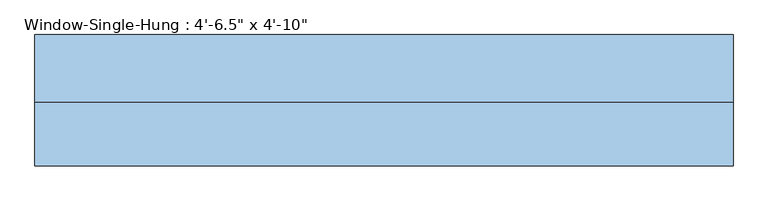
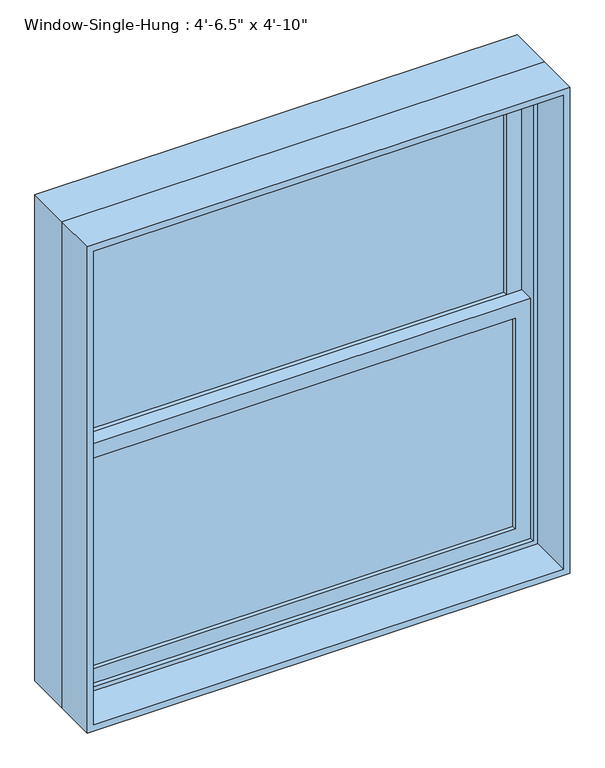
"""IFC4 building model written with IfcOpenShell, lengths in millimetres: window geometry."""

import ifcopenshell
import ifcopenshell.guid

model = None  # the IFC model being written
_history = None  # IfcOwnerHistory: only IFC2X3 demands one
_inside = {}  # id of a spatial element -> (the spatial element, [elements in it])
_under = {}  # id of a project, library or spatial element -> (it, [spatial elements below it])
_declared = {}  # id of a project -> (the project, [libraries it declares])
_typed = {}  # id of a type object -> (the type object, [elements of that type])
_made_of = {}  # id of a material, layer set ... -> (it, [elements and type objects made of it])


def new_model(schema):
    """Start an empty IFC model of exactly this schema.

    Asked for "IFC4X3", IfcOpenShell would pick the latest addendum, in which some entities
    have other attributes; the version numbers below select the first issue.
    IFC2X3 requires an IfcOwnerHistory on every rooted entity: one is made here for all.
    """
    global model, _history
    if schema == "IFC4X3":
        model = ifcopenshell.file(schema_version=(4, 3, 0, 0))
    else:
        model = ifcopenshell.file(schema=schema)
    _inside.clear()
    _under.clear()
    _declared.clear()
    _typed.clear()
    _made_of.clear()
    _history = None
    if model.schema == "IFC2X3":
        org = make("IfcOrganization", Name="unknown")
        user = make(
            "IfcPersonAndOrganization",
            ThePerson=make("IfcPerson", FamilyName="unknown"),
            TheOrganization=org,
        )
        app = make(
            "IfcApplication",
            ApplicationDeveloper=org,
            Version="unknown",
            ApplicationFullName="unknown",
            ApplicationIdentifier="unknown",
        )
        _history = make(
            "IfcOwnerHistory",
            OwningUser=user,
            OwningApplication=app,
            ChangeAction="ADDED",
            CreationDate=0,
        )
    return model


def make(cls, **values):
    """One entity of the class cls with the attributes given. An attribute that is None is left unset."""
    return model.create_entity(
        cls, **{name: value for name, value in values.items() if value is not None}
    )


def rooted(cls, **values):
    """An entity with a GlobalId (a new one), such as an element, a storey or a relation."""
    return make(cls, GlobalId=ifcopenshell.guid.new(), OwnerHistory=_history, **values)


def si_unit(unit_type, name, prefix=None):
    """IfcSIUnit, for example si_unit("LENGTHUNIT", "METRE", prefix="MILLI")."""
    return make("IfcSIUnit", UnitType=unit_type, Prefix=prefix, Name=name)


def assignment(units):
    """IfcUnitAssignment: the units of a project."""
    return None if units is None else make("IfcUnitAssignment", Units=units)


def point(xyz):
    """IfcCartesianPoint."""
    return None if xyz is None else make("IfcCartesianPoint", Coordinates=xyz)


def direction(xyz):
    """IfcDirection."""
    return None if xyz is None else make("IfcDirection", DirectionRatios=xyz)


def frame(location, z_axis=None, x_axis=None):
    """IfcAxis2Placement3D, a coordinate frame: its origin and axes. An axis left out is left unset."""
    return make(
        "IfcAxis2Placement3D",
        Location=point(location),
        Axis=direction(z_axis),
        RefDirection=direction(x_axis),
    )


def origin():
    """The frame at (0, 0, 0) with its axes left unset."""
    return frame((0.0, 0.0, 0.0))


def place(relative_to, where):
    """IfcLocalPlacement: puts the frame where relative to a parent placement (None: the world)."""
    return make(
        "IfcLocalPlacement", PlacementRelTo=relative_to, RelativePlacement=where
    )


def context(
    kind, dimensions, precision=None, world=None, true_north=None, identifier=None
):
    """IfcGeometricRepresentationContext, for example the 3D "Model" context."""
    return make(
        "IfcGeometricRepresentationContext",
        ContextIdentifier=identifier,
        ContextType=kind,
        CoordinateSpaceDimension=dimensions,
        Precision=precision,
        WorldCoordinateSystem=world,
        TrueNorth=true_north,
    )


def project(units=None, contexts=None):
    """IfcProject with its units and contexts."""
    return rooted(
        "IfcProject",
        Name="project",
        RepresentationContexts=contexts,
        UnitsInContext=assignment(units),
    )


def spatial(cls, under=None, at=None, **own):
    """A site, building, storey or space (cls), placed at a placement, below another one or the project."""
    s = rooted(cls, ObjectPlacement=at, **own)
    if under is not None:
        _under.setdefault(under.id(), (under, []))[1].append(s)
    return s


def polyline(points):
    """IfcPolyline through the points."""
    return make("IfcPolyline", Points=[point(p) for p in points])


def outline(outer, holes=None, kind="AREA"):
    """IfcArbitraryClosedProfileDef: a profile drawn as a closed curve; with holes, ...WithVoids."""
    if holes is None:
        return make("IfcArbitraryClosedProfileDef", ProfileType=kind, OuterCurve=outer)
    return make(
        "IfcArbitraryProfileDefWithVoids",
        ProfileType=kind,
        OuterCurve=outer,
        InnerCurves=holes,
    )


def extrude(swept, where, along, depth):
    """IfcExtrudedAreaSolid: the profile swept, set in the frame where, extruded along a direction by depth."""
    return make(
        "IfcExtrudedAreaSolid",
        SweptArea=swept,
        Position=where,
        ExtrudedDirection=direction(along),
        Depth=depth,
    )


def shape(context_of_items, identifier, shape_type, items):
    """IfcShapeRepresentation: the items that make up one representation, for example the "Body"."""
    return make(
        "IfcShapeRepresentation",
        ContextOfItems=context_of_items,
        RepresentationIdentifier=identifier,
        RepresentationType=shape_type,
        Items=items,
    )


def source(mapping_origin, context_of_items, identifier, shape_type, items):
    """IfcRepresentationMap: a shape defined once, which mapped items show again and again."""
    return make(
        "IfcRepresentationMap",
        MappingOrigin=mapping_origin,
        MappedRepresentation=shape(context_of_items, identifier, shape_type, items),
    )


def transform(
    local_origin,
    x_axis=None,
    y_axis=None,
    z_axis=None,
    scale=None,
    scale2=None,
    scale3=None,
    uniform=True,
):
    """IfcCartesianTransformationOperator3D, or its non-uniform kind. x_axis, y_axis, z_axis: its Axis1, 2, 3."""
    if uniform:
        return make(
            "IfcCartesianTransformationOperator3D",
            Axis1=direction(x_axis),
            Axis2=direction(y_axis),
            LocalOrigin=point(local_origin),
            Scale=scale,
            Axis3=direction(z_axis),
        )
    return make(
        "IfcCartesianTransformationOperator3DnonUniform",
        Axis1=direction(x_axis),
        Axis2=direction(y_axis),
        LocalOrigin=point(local_origin),
        Scale=scale,
        Axis3=direction(z_axis),
        Scale2=scale2,
        Scale3=scale3,
    )


def mapped(mapping_source, mapping_target):
    """IfcMappedItem: shows the shape of a source again, moved by a transform."""
    return make(
        "IfcMappedItem", MappingSource=mapping_source, MappingTarget=mapping_target
    )


def made_of(thing, what):
    """Note that an element or type object is made of a material, layer set ...; save() writes the relation."""
    if what is not None:
        _made_of.setdefault(what.id(), (what, []))[1].append(thing)
    return thing


def element(
    cls,
    number,
    at=None,
    inside=None,
    cuts=None,
    type_object=None,
    material=None,
    context=None,
    identifier="Body",
    shape_type=None,
    held_by="IfcProductDefinitionShape",
    body=None,
    shapes=None,
    **own,
):
    """One element of the class cls, such as IfcWall. Its Tag is "e" and its number.

    at: its placement. inside: the storey or other place that contains it. cuts: it is an
    opening in that element (IfcRelVoidsElement). A single representation is given by context,
    identifier, shape_type and body (its items); several are given by shapes. held_by: the class
    of the entity that holds the representations. save() writes the other relations.
    """
    e = rooted(cls, Tag="e%d" % number, ObjectPlacement=at, **own)
    if body is not None:
        shapes = [shape(context, identifier, shape_type, body)]
    if shapes is not None:
        e.Representation = make(held_by, Representations=shapes)
    if inside is not None:
        _inside.setdefault(inside.id(), (inside, []))[1].append(e)
    if cuts is not None:
        rooted(
            "IfcRelVoidsElement", RelatingBuildingElement=cuts, RelatedOpeningElement=e
        )
    if type_object is not None:
        _typed.setdefault(type_object.id(), (type_object, []))[1].append(e)
    return made_of(e, material)


def aggregate(whole, parts):
    """IfcRelAggregates: a whole, such as a stair, and the parts it consists of."""
    return rooted("IfcRelAggregates", RelatingObject=whole, RelatedObjects=parts)


def save(model, path):
    """Write the relations noted so far, then the file.

    IfcRelAggregates (storeys below a building ...), IfcRelContainedInSpatialStructure (elements
    in a storey), IfcRelDefinesByType, IfcRelAssociatesMaterial and IfcRelDeclares: one each for
    every whole, place, type object, material and project.
    """
    for whole, parts in _under.values():
        aggregate(whole, parts)
    for where, things in _inside.values():
        rooted(
            "IfcRelContainedInSpatialStructure",
            RelatedElements=things,
            RelatingStructure=where,
        )
    for kind, things in _typed.values():
        rooted("IfcRelDefinesByType", RelatedObjects=things, RelatingType=kind)
    for what, things in _made_of.values():
        rooted("IfcRelAssociatesMaterial", RelatedObjects=things, RelatingMaterial=what)
    for by, libraries in _declared.values():
        rooted("IfcRelDeclares", RelatingContext=by, RelatedDefinitions=libraries)
    model.write(path)


def window_bd35b4c6(model_context):
    return source(origin(), model_context, "Body", "SweptSolid", [
        extrude(outline(polyline([(615.95, 50.8), (615.95, 44.45), (-615.95, 44.45), (-615.95, 50.8), (615.95, 50.8)])), frame((0.0, 0.0, 990.6), z_axis=(0.0, 0.0, 1.0), x_axis=(1.0, 0.0, 0.0)), (0.0, 0.0, 1.0), 638.175),
        extrude(outline(polyline([(-615.95, 38.1), (615.95, 38.1), (615.95, 31.75), (-615.95, 31.75), (-615.95, 38.1)])), frame((0.0, 0.0, 990.6), z_axis=(0.0, 0.0, 1.0), x_axis=(1.0, 0.0, 0.0)), (0.0, 0.0, 1.0), 638.175),
        extrude(outline(polyline([(615.95, 95.25), (615.95, 88.9), (-615.95, 88.9), (-615.95, 95.25), (615.95, 95.25)])), frame((0.0, 0.0, 1673.225), z_axis=(0.0, 0.0, 1.0), x_axis=(1.0, 0.0, 0.0)), (0.0, 0.0, 1.0), 638.175),
        extrude(outline(polyline([(-615.95, 82.55), (615.95, 82.55), (615.95, 76.2), (-615.95, 76.2), (-615.95, 82.55)])), frame((0.0, 0.0, 1673.225), z_axis=(0.0, 0.0, 1.0), x_axis=(1.0, 0.0, 0.0)), (0.0, 0.0, 1.0), 638.175),
        extrude(outline(polyline([(1673.225, -660.4), (946.15, -660.4), (946.15, 660.4), (1673.225, 660.4), (1673.225, -660.4)]), holes=[polyline([(1628.775, 615.95), (990.6, 615.95), (990.6, -615.95), (1628.775, -615.95), (1628.775, 615.95)])]), frame((0.0, 19.05, 0.0), z_axis=(0.0, 1.0, 0.0), x_axis=(0.0, 0.0, 1.0)), (0.0, 0.0, 1.0), 44.45),
        extrude(outline(polyline([(2355.85, -660.4), (1628.775, -660.4), (1628.775, 660.4), (2355.85, 660.4), (2355.85, -660.4)]), holes=[polyline([(2311.4, 615.95), (1673.225, 615.95), (1673.225, -615.95), (2311.4, -615.95), (2311.4, 615.95)])]), frame((0.0, 63.5, 0.0), z_axis=(0.0, 1.0, 0.0), x_axis=(0.0, 0.0, 1.0)), (0.0, 0.0, 1.0), 44.45),
        extrude(outline(polyline([(2387.6, -692.15), (914.4, -692.15), (914.4, 692.15), (2387.6, 692.15), (2387.6, -692.15)]), holes=[polyline([(2355.85, 660.4), (946.15, 660.4), (946.15, -660.4), (2355.85, -660.4), (2355.85, 660.4)])]), frame((0.0, 6.35, 0.0), z_axis=(0.0, 1.0, 0.0), x_axis=(0.0, 0.0, 1.0)), (0.0, 0.0, 1.0), 133.35),
        extrude(outline(polyline([(2387.6, 692.15), (2387.6, -692.15), (914.4, -692.15), (914.4, 692.15), (2387.6, 692.15)]), holes=[polyline([(2368.55, 673.1), (933.45, 673.1), (933.45, -673.1), (2368.55, -673.1), (2368.55, 673.1)])]), frame((0.0, -120.65, 0.0), z_axis=(0.0, 1.0, 0.0), x_axis=(0.0, 0.0, 1.0)), (0.0, 0.0, 1.0), 127.0),
    ])


if __name__ == "__main__":
    model = new_model("IFC4")
    model_context = context("Model", 3, world=origin())
    ifc_project = project(units=[si_unit("LENGTHUNIT", "METRE", prefix="MILLI")], contexts=[model_context])
    site = spatial("IfcSite", under=ifc_project)
    building = spatial("IfcBuilding", under=site)
    placement = place(None, origin())
    window_shape = window_bd35b4c6(model_context)
    element("IfcWindow", 1, ObjectType="Window-Single-Hung : 4'-6.5\" x 4'-10\"", at=placement, inside=building, context=model_context, shape_type="MappedRepresentation", body=[
        mapped(window_shape, transform((0.0, 0.0, 0.0), x_axis=(1.0, 0.0, 0.0), y_axis=(0.0, 1.0, 0.0), z_axis=(0.0, 0.0, 1.0))),
    ])
    save(model, "model.ifc")

# Revit data of these elements
# Type "Window-Single-Hung : 4'-6.5\" x 4'-10\""
#   Type Mark = "28"
#   Fire Rating = "0.5h"
#   Construction Type Id = "DG-DR"
#   Assembly Code = "B2020100"
#   Analytic Construction = "Double glazing - domestic"
#   Wall Thickness [instance default] = 0' - 6"
#   Window Inset [instance default] = 0' - 0"
#   Visual Light Transmittance = 0.81
#   Thermal Resistance (R) = 0.319569 (m²·K)/W
#   Solar Heat Gain Coefficient = 0.76
#   Muntin Width = 4' - 0 1/2"
#   Muntin Height = 2' - 1 1/8"
#   Interior Wall Closure [instance default] = 0' - 1 1/2"
#   Rough Width = 4' - 7"
#   Rough Height = 4' - 10 1/2"
#   Frame Extension [instance default] = 0' - 1 1/4"
#   Exterior Wall Closure [instance default] = 0' - 0 1/2"
#   Extension Jamb [instance default] = 0' - 1 1/2"
#   Heat Transfer Coefficient (U) = 3.12929 W/(m²·K)
#   Height = 4' - 10"
#   Width = 4' - 6 1/2"
#   Top Muntin Visibility = yes
#   Indicator Visibility [instance default] = yes
#   Extension Jamb Visibility [instance default] = yes
#   Interior Trim Visibility [instance default] = yes
#   Exterior Trim Visibility [instance default] = yes
#   Bottom Muntin Visibility = yes
#   Muntin Pattern = Muntin Pattern_2x2 : Muntin Pattern_2x2
#   Interior Trim Material = Wood - Stained
#   Interior Trim = Trim-Window-Interior-Flat : Picture Frame
#   Exterior Trim Material = Clad - White
#   Exterior Trim = Trim-Window-Exterior-Flat : with Sill
#   Glass Panel Material = Glass
#   Exterior Frame Material = Clad - White
#   Interior Frame Material = Wood - Stained
#   Wall Closure = (empty or 0)
# Element 1 (IfcWindow, "Window-Single-Hung : 4'-6.5\" x 4'-10\"")
#   Wall Thickness = 0' - 9 1/2"
#   Extension Jamb = 0' - 5"
#   Materials on its faces: "Wood - Stained", "Glass", "Clad - White"
# Materials
#   "Wood - Stained": class "Wood", colour RGB 224 178 126, transparency 0, Cost = 0
#   "Clad - White": class "Wood", colour RGB 242 242 238, transparency 0, Cost = 0
#   "Glass": class "Glass", colour RGB 218 227 224, transparency 0.85, Description = "Soda Lime Glass", Cost = 0
